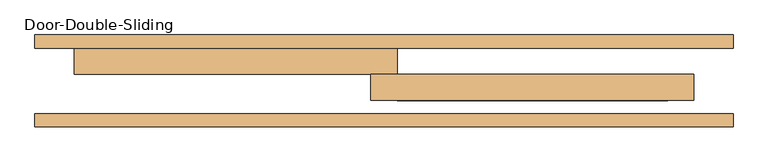
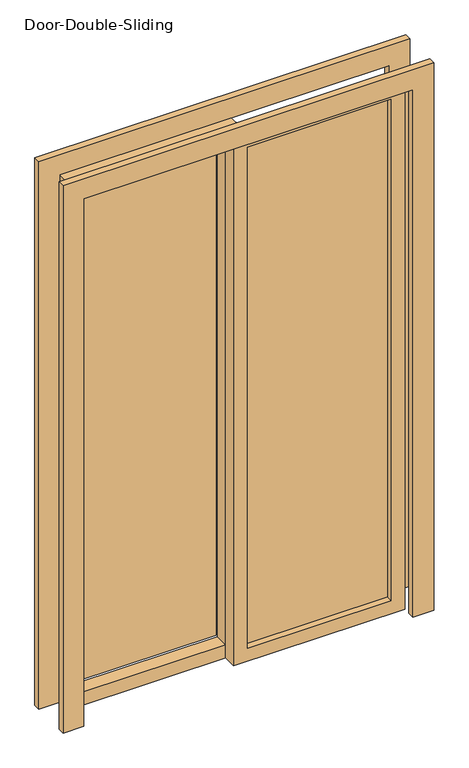
"""IFC4 building model written with IfcOpenShell, lengths in millimetres: door geometry, Door-Double-Sliding : CUARTO."""

from ifc_helpers import new_model, si_unit, frame, origin, place, context, project, spatial, polyline, outline, extrude, source, transform, mapped, element, save


def door_double_sliding_e8ceb126(model_context):
    return source(origin(), model_context, "Body", "SweptSolid", [
        extrude(outline(polyline([(0.0, -676.2), (0.0, -600.0), (2032.0, -600.0), (2032.0, 600.0), (0.0, 600.0), (0.0, 676.2), (2108.2, 676.2), (2108.2, -676.2), (0.0, -676.2)])), frame((0.0, 38.1, 0.0), z_axis=(0.0, 1.0, 0.0), x_axis=(0.0, 0.0, 1.0)), (0.0, 0.0, 1.0), 25.4),
        extrude(outline(polyline([(0.0, 676.2), (2108.2, 676.2), (2108.2, -676.2), (0.0, -676.2), (0.0, -600.0), (2032.0, -600.0), (2032.0, 600.0), (0.0, 600.0), (0.0, 676.2)])), frame((0.0, 190.5, 0.0), z_axis=(0.0, 1.0, 0.0), x_axis=(0.0, 0.0, 1.0)), (0.0, 0.0, 1.0), 25.4),
        extrude(outline(polyline([(2032.0, -25.4), (0.0, -25.4), (0.0, 600.0), (2032.0, 600.0), (2032.0, -25.4)]), holes=[polyline([(1981.2, 25.4), (1981.2, 549.2), (50.8, 549.2), (50.8, 25.4), (1981.2, 25.4)])]), frame((0.0, 88.9, 0.0), z_axis=(0.0, 1.0, 0.0), x_axis=(0.0, 0.0, 1.0)), (0.0, 0.0, 1.0), 50.8),
        extrude(outline(polyline([(2032.0, 25.4), (2032.0, -600.0), (0.0, -600.0), (0.0, 25.4), (2032.0, 25.4)]), holes=[polyline([(1981.2, -25.4), (50.8, -25.4), (50.8, -549.2), (1981.2, -549.2), (1981.2, -25.4)])]), frame((0.0, 139.7, 0.0), z_axis=(0.0, 1.0, 0.0), x_axis=(0.0, 0.0, 1.0)), (0.0, 0.0, 1.0), 50.8),
        extrude(outline(polyline([(25.4, 117.475), (549.2, 117.475), (549.2, 111.125), (25.4, 111.125), (25.4, 117.475)])), frame((0.0, 0.0, 50.8), z_axis=(0.0, 0.0, 1.0), x_axis=(1.0, 0.0, 0.0)), (0.0, 0.0, 1.0), 1930.4),
        extrude(outline(polyline([(-25.4, 200.025), (-549.2, 200.025), (-549.2, 206.375), (-25.4, 206.375), (-25.4, 200.025)])), frame((0.0, 0.0, 50.8), z_axis=(0.0, 0.0, 1.0), x_axis=(1.0, 0.0, 0.0)), (0.0, 0.0, 1.0), 1930.4),
    ])


if __name__ == "__main__":
    model = new_model("IFC4")
    model_context = context("Model", 3, world=origin())
    ifc_project = project(units=[si_unit("LENGTHUNIT", "METRE", prefix="MILLI")], contexts=[model_context])
    site = spatial("IfcSite", under=ifc_project)
    building = spatial("IfcBuilding", under=site)
    placement = place(None, origin())
    door_double_sliding_shape = door_double_sliding_e8ceb126(model_context)
    element("IfcDoor", 1, ObjectType="Door-Double-Sliding : CUARTO", at=placement, inside=building, context=model_context, shape_type="MappedRepresentation", body=[
        mapped(door_double_sliding_shape, transform((0.0, 0.0, 0.0), x_axis=(1.0, 0.0, 0.0), y_axis=(0.0, 1.0, 0.0), z_axis=(0.0, 0.0, 1.0))),
    ])
    save(model, "model.ifc")

# Revit data of these elements
# Type "Door-Double-Sliding : CUARTO"
#   Type Mark = "10"
#   Construction Type Id = "opn-d45"
#   Assembly Code = "C1020"
#   Analytic Construction = "Wood frame, double glass door "
#   Thickness = 0.0508 m
#   Thermal Resistance (R) = 0.31964 (m²·K)/W
#   Heat Transfer Coefficient (U) = 3.12872 W/(m²·K)
#   Height = 2.032 m
#   Rail Width = 0.0508 m
#   Stiles = 0.0508 m
#   Trim Projection Ext = 0.0254 m
#   Trim Projection Int = 0.0254 m
#   Trim Width = 0.0762 m
#   Width = 1.20 m
#   Glazing = Glass
#   Panel Material = Wood - Birch - Solid Stained Light Low Gloss
#   Trim Material = Paint - Sienna
#   Visual Light Transmittance = 0
#   Solar Heat Gain Coefficient = 0
#   Function = (empty or 0)
#   Wall Closure = (empty or 0)
# Element 1 (IfcDoor, "Door-Double-Sliding : CUARTO")
#   Materials on its faces: "Paint - Sienna", "Wood - Birch - Solid Stained Light Low Gloss", "Glass"
# Materials
#   "Glass": class "Glass", colour RGB 213 204 197, transparency 0.85, Description = "Soda Lime Glass", Cost = 0
#   "Wood - Birch - Solid Stained Light Low Gloss": class "Wood", colour RGB 227 170 128, transparency 0, Cost = 0
#   "Paint - Sienna": class "Miscellaneous", colour RGB 118 70 51, transparency 0, Cost = 0
